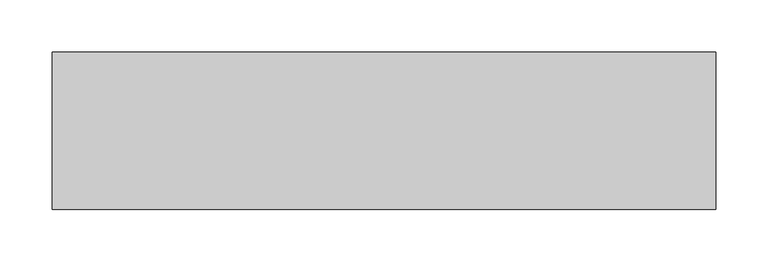
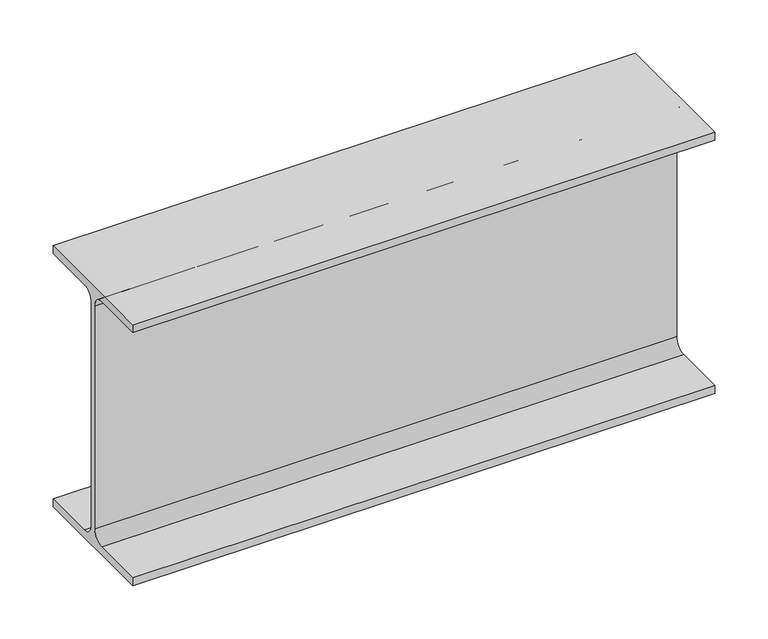
"""IFC4 building model written with IfcOpenShell, lengths in millimetres: beam geometry, 0912_Steel Framing_H-KSD3502 : H_SB_ASB_H-300x150x6.5x9."""

from ifc_helpers import new_model, si_unit, point, frame, frame_2d, origin, place, context, project, spatial, polyline, circle_curve, trimmed, segment, composite_curve, outline, extrude, source, transform, mapped, element, save


def beam_2895a1d0(model_context):
    return source(origin(), model_context, "Body", "SweptSolid", [
        extrude(outline(composite_curve([segment(polyline([(75.0, -141.0), (75.0, -150.0), (-75.0, -150.0), (-75.0, -141.0), (-16.25, -141.0)]), True, "CONTINUOUS"), segment(trimmed(circle_curve(frame_2d((-16.25, -128.0)), 13.0), [point((-16.25, -141.0))], [point((-3.25, -128.0))], True, "CARTESIAN"), True, "CONTINUOUS"), segment(polyline([(-3.25, -128.0), (-3.25, 128.0)]), True, "CONTINUOUS"), segment(trimmed(circle_curve(frame_2d((-16.25, 128.0)), 13.0), [point((-3.25, 128.0))], [point((-16.25, 141.0))], True, "CARTESIAN"), True, "CONTINUOUS"), segment(polyline([(-16.25, 141.0), (-75.0, 141.0), (-75.0, 150.0), (75.0, 150.0), (75.0, 141.0), (16.25, 141.0)]), True, "CONTINUOUS"), segment(trimmed(circle_curve(frame_2d((16.25, 128.0)), 13.0), [point((16.25, 141.0))], [point((3.25, 128.0))], True, "CARTESIAN"), True, "CONTINUOUS"), segment(polyline([(3.25, 128.0), (3.25, -128.0)]), True, "CONTINUOUS"), segment(trimmed(circle_curve(frame_2d((16.25, -128.0)), 13.0), [point((3.25, -128.0))], [point((16.25, -141.0))], True, "CARTESIAN"), True, "CONTINUOUS"), segment(polyline([(16.25, -141.0), (75.0, -141.0)]), True, "CONTINUOUS")], self_intersect=False)), frame((-282.3, 0.0, 0.0), z_axis=(1.0, 0.0, 0.0), x_axis=(0.0, 1.0, 0.0)), (0.0, 0.0, 1.0), 632.1),
    ])


if __name__ == "__main__":
    model = new_model("IFC4")
    model_context = context("Model", 3, world=origin())
    ifc_project = project(units=[si_unit("LENGTHUNIT", "METRE", prefix="MILLI")], contexts=[model_context])
    site = spatial("IfcSite", under=ifc_project)
    building = spatial("IfcBuilding", under=site)
    placement = place(None, origin())
    beam_shape = beam_2895a1d0(model_context)
    element("IfcBeam", 1, ObjectType="0912_Steel Framing_H-KSD3502 : H_SB_ASB_H-300x150x6.5x9", at=placement, inside=building, context=model_context, shape_type="MappedRepresentation", body=[
        mapped(beam_shape, transform((0.0, 0.0, 0.0), x_axis=(1.0, 0.0, 0.0), y_axis=(0.0, 1.0, 0.0), z_axis=(0.0, 0.0, 1.0))),
    ])
    save(model, "model.ifc")

# Revit data of these elements
# Type "0912_Steel Framing_H-KSD3502 : H_SB_ASB_H-300x150x6.5x9"
#   H_WM Code_1 = "S01AA002-00001 | Main Steel Structure Fabrication Work | Shelter/Building | Medium Steel - Standard (90KG/M>Weight≥30KG/M) | Material: (   )"
#   H_WM Code_2 = "S03AA028-00001 | Main Steel Structure Erection Work | Shelter/Building | Medium Steel (90KG/M>Weight≥30KG/M) | Material: (   )"
#   H_WM Code_3 = "S01AA010-00001 | Main Steel Structure Fabrication Work | Shelter/Building | Steel Painting/Coating | for Non-Fireproofed Steel Surface, Surface Preparation, Primer, Second & Final Coat | Material: (   )"
#   H_Q'ty Cal Type Tag = "SB-Q2"
#   Width = 15.0 cm
#   Web Thickness = 0.65 cm
#   Web Fillet = 1.3 cm
#   Warping Constant = 107000.0 cm⁶
#   W = 0
#   Torsional Moment of Inertia = 9.9539 cm⁴
#   Section Area = 46.78 cm²
#   Plastic Modulus weak axis = 105.0 cm³
#   Plastic Modulus strong axis = 542.0 cm³
#   Perimeter = 1.17 m²/m
#   Nominal Weight = 36.70 kgf/m
#   Moment of Inertia weak axis = 508.00 cm⁴
#   Moment of Inertia strong axis = 7210.00 cm⁴
#   Height = 30.0 cm
#   Flange Thickness = 0.9 cm
#   Elastic Modulus weak axis = 67.7 cm³
#   Elastic Modulus strong axis = 481.0 cm³
#   Centroid Vertical = 15.0 cm
#   Centroid Horizontal = 7.5 cm
#   Ix = 72100000
#   Length [instance default] = 1.5240 m
#   Zx = 542000
#   b = 0.1500 m
#   h = 0.3000 m
#   r = 0.0130 m
#   s = 0.0065 m
#   t = 0.0090 m
#   A = 0.004678 m²
#   Structural Material [instance default] = Steel, 45-345
#   Assembly Code = ""
# Element 1 (IfcBeam, "0912_Steel Framing_H-KSD3502 : H_SB_ASB_H-300x150x6.5x9")
#   Structural Material = none
# Materials
#   "Steel, 45-345": class "Metal", colour RGB 189 187 185, transparency 0, Description = "Steel 345 MPa", Cost = 0
